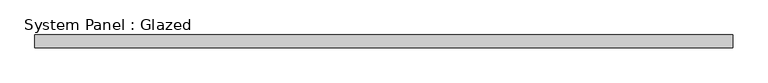
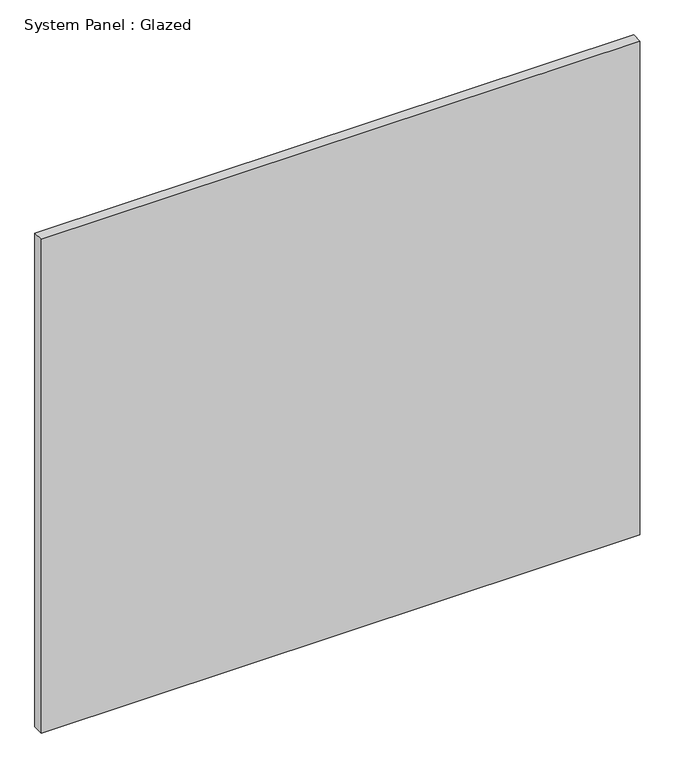
"""IFC4 building model written with IfcOpenShell, lengths in millimetres: plate geometry, System Panel : Glazed."""

from ifc_helpers import new_model, si_unit, origin, origin_with_axes, place, context, project, spatial, polyline, outline, extrude, source, transform, mapped, element, save


def system_panel_glazed_09ad70ba(model_context):
    return source(origin(), model_context, "Body", "SweptSolid", [
        extrude(outline(polyline([(688.1363635, 24.5), (-688.1363635, 24.5), (-688.1363635, 49.5), (688.1363635, 49.5), (688.1363635, 24.5)])), origin_with_axes(), (0.0, 0.0, 1.0), 1200.0),
    ])


if __name__ == "__main__":
    model = new_model("IFC4")
    model_context = context("Model", 3, world=origin())
    ifc_project = project(units=[si_unit("LENGTHUNIT", "METRE", prefix="MILLI")], contexts=[model_context])
    site = spatial("IfcSite", under=ifc_project)
    building = spatial("IfcBuilding", under=site)
    placement = place(None, origin())
    system_panel_glazed_shape = system_panel_glazed_09ad70ba(model_context)
    element("IfcPlate", 1, ObjectType="System Panel : Glazed", at=placement, inside=building, context=model_context, shape_type="MappedRepresentation", body=[
        mapped(system_panel_glazed_shape, transform((0.0, 0.0, 0.0), x_axis=(1.0, 0.0, 0.0), y_axis=(0.0, 1.0, 0.0), z_axis=(0.0, 0.0, 1.0))),
    ])
    save(model, "model.ifc")

# Revit data of these elements
# Element 1 (IfcPlate, "System Panel : Glazed")
#   Materials on its faces: "Glass"
# Materials
#   "Glass": class "Glass", colour RGB 218 227 224, transparency 0.85, Description = "Soda Lime Glass", Cost = 0
